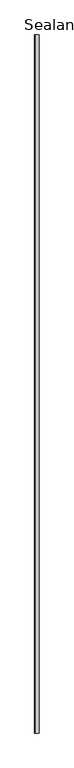
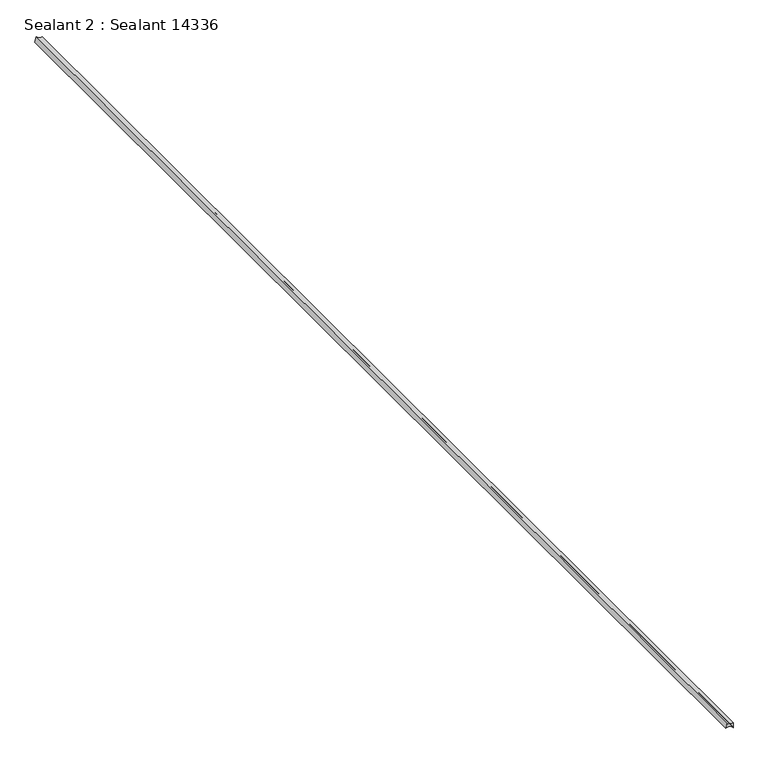
"""IFC4 building model written with IfcOpenShell, lengths in millimetres: proxy geometry, Sealant 2 : Sealant 14336."""

from ifc_helpers import new_model, si_unit, point, frame, frame_2d, origin, place, context, project, spatial, polyline, circle_curve, trimmed, segment, composite_curve, outline, extrude, source, transform, mapped, element, save


def sealant_2_sealant_14336_31959efe(model_context):
    return source(origin(), model_context, "Body", "SweptSolid", [
        extrude(outline(composite_curve([segment(polyline([(43747.9055798, 5326.5479115), (43739.432414, 5323.9245492)]), True, "CONTINUOUS"), segment(trimmed(circle_curve(frame_2d((43732.4637088, 5328.9062913)), 8.5662482), [point((43739.432414, 5323.9245492))], [point((43736.5432875, 5336.4387308))], True, "CARTESIAN"), True, "CONTINUOUS"), segment(polyline([(43736.5432875, 5336.4387308), (43744.7831609, 5336.4387308)]), True, "CONTINUOUS"), segment(trimmed(circle_curve(frame_2d((43754.3961889, 5334.0351885)), 9.9089516), [point((43744.7831609, 5336.4387308))], [point((43747.9055798, 5326.5479115))], True, "CARTESIAN"), True, "CONTINUOUS")], self_intersect=False)), frame((0.0, -1052.8906574, 0.0), z_axis=(0.0, 1.0, 0.0), x_axis=(0.0, 0.0, 1.0)), (0.0, 0.0, 1.0), 1999.85),
    ])


if __name__ == "__main__":
    model = new_model("IFC4")
    model_context = context("Model", 3, world=origin())
    ifc_project = project(units=[si_unit("LENGTHUNIT", "METRE", prefix="MILLI")], contexts=[model_context])
    site = spatial("IfcSite", under=ifc_project)
    building = spatial("IfcBuilding", under=site)
    placement = place(None, origin())
    sealant_2_sealant_14336_shape = sealant_2_sealant_14336_31959efe(model_context)
    element("IfcBuildingElementProxy", 1, Name="Sealant 2 : Sealant 14336", ObjectType="Sealant 2 : Sealant 14336", at=placement, inside=building, context=model_context, shape_type="MappedRepresentation", body=[
        mapped(sealant_2_sealant_14336_shape, transform((0.0, 0.0, 0.0), x_axis=(1.0, 0.0, 0.0), y_axis=(0.0, 1.0, 0.0), z_axis=(0.0, 0.0, 1.0))),
    ])
    save(model, "model.ifc")

# Revit data of these elements
# Type "Sealant 2 : Sealant 14336"
#   NameOverride = "Sealant"
# Element 1 (IfcBuildingElementProxy, "Sealant 2 : Sealant 14336")
#   Materials on its faces: "SEALANT AND BACKER ROD WHERE NECESSARY"
# Materials
#   "SEALANT AND BACKER ROD WHERE NECESSARY": class "Unassigned", colour RGB 225 240 198, transparency 0, Cost = 0
